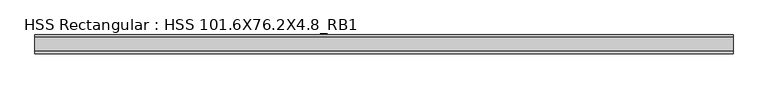
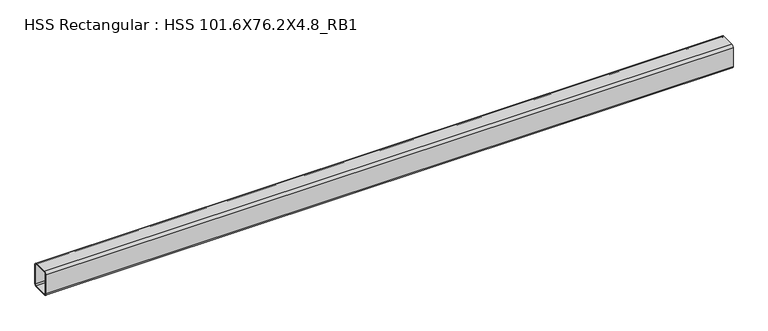
"""IFC4 building model written with IfcOpenShell, lengths in millimetres: beam geometry, HSS Rectangular : HSS 101.6X76.2X4.8_RB1."""

from ifc_helpers import new_model, si_unit, point, frame, frame_2d, origin, place, context, project, spatial, polyline, circle_curve, trimmed, segment, composite_curve, outline, extrude, source, transform, mapped, element, save


def hss_rectangular_hss_101_6x76_2x4_8_rb1_1d8725ce(model_context):
    return source(origin(), model_context, "Body", "SweptSolid", [
        extrude(outline(composite_curve([segment(trimmed(circle_curve(frame_2d((-28.575, 41.275)), 9.525), [point((-38.1, 41.275))], [point((-28.575, 50.8))], False, "CARTESIAN"), True, "CONTINUOUS"), segment(polyline([(-28.575, 50.8), (28.575, 50.8)]), True, "CONTINUOUS"), segment(trimmed(circle_curve(frame_2d((28.575, 41.275)), 9.525), [point((28.575, 50.8))], [point((38.1, 41.275))], False, "CARTESIAN"), True, "CONTINUOUS"), segment(polyline([(38.1, 41.275), (38.1, -41.275)]), True, "CONTINUOUS"), segment(trimmed(circle_curve(frame_2d((28.575, -41.275)), 9.525), [point((38.1, -41.275))], [point((28.575, -50.8))], False, "CARTESIAN"), True, "CONTINUOUS"), segment(polyline([(28.575, -50.8), (-28.575, -50.8)]), True, "CONTINUOUS"), segment(trimmed(circle_curve(frame_2d((-28.575, -41.275)), 9.525), [point((-28.575, -50.8))], [point((-38.1, -41.275))], False, "CARTESIAN"), True, "CONTINUOUS"), segment(polyline([(-38.1, -41.275), (-38.1, 41.275)]), True, "CONTINUOUS")], self_intersect=False), holes=[composite_curve([segment(polyline([(28.575, 46.0375), (-28.575, 46.0375)]), True, "CONTINUOUS"), segment(trimmed(circle_curve(frame_2d((-28.575, 41.275)), 4.7625), [point((-28.575, 46.0375))], [point((-33.3375, 41.275))], True, "CARTESIAN"), True, "CONTINUOUS"), segment(polyline([(-33.3375, 41.275), (-33.3375, -41.275)]), True, "CONTINUOUS"), segment(trimmed(circle_curve(frame_2d((-28.575, -41.275)), 4.7625), [point((-33.3375, -41.275))], [point((-28.575, -46.0375))], True, "CARTESIAN"), True, "CONTINUOUS"), segment(polyline([(-28.575, -46.0375), (28.575, -46.0375)]), True, "CONTINUOUS"), segment(trimmed(circle_curve(frame_2d((28.575, -41.275)), 4.7625), [point((28.575, -46.0375))], [point((33.3375, -41.275))], True, "CARTESIAN"), True, "CONTINUOUS"), segment(polyline([(33.3375, -41.275), (33.3375, 41.275)]), True, "CONTINUOUS"), segment(trimmed(circle_curve(frame_2d((28.575, 41.275)), 4.7625), [point((33.3375, 41.275))], [point((28.575, 46.0375))], True, "CARTESIAN"), True, "CONTINUOUS")], self_intersect=False)]), frame((-1442.3750006, 0.0, 0.0), z_axis=(1.0, 0.0, 0.0), x_axis=(0.0, 1.0, 0.0)), (0.0, 0.0, 1.0), 2827.6000006),
    ])


if __name__ == "__main__":
    model = new_model("IFC4")
    model_context = context("Model", 3, world=origin())
    ifc_project = project(units=[si_unit("LENGTHUNIT", "METRE", prefix="MILLI")], contexts=[model_context])
    site = spatial("IfcSite", under=ifc_project)
    building = spatial("IfcBuilding", under=site)
    placement = place(None, origin())
    hss_rectangular_hss_101_6x76_2x4_8_rb1_shape = hss_rectangular_hss_101_6x76_2x4_8_rb1_1d8725ce(model_context)
    element("IfcBeam", 1, ObjectType="HSS Rectangular : HSS 101.6X76.2X4.8_RB1", at=placement, inside=building, context=model_context, shape_type="MappedRepresentation", body=[
        mapped(hss_rectangular_hss_101_6x76_2x4_8_rb1_shape, transform((0.0, 0.0, 0.0), x_axis=(1.0, 0.0, 0.0), y_axis=(0.0, 1.0, 0.0), z_axis=(0.0, 0.0, 1.0))),
    ])
    save(model, "model.ifc")

# Revit data of these elements
# Type "HSS Rectangular : HSS 101.6X76.2X4.8_RB1"
#   Section Name Key = "HSS 4X3X3/16"
#   Assembly Code = "B10"
#   Width = 7.62 cm
#   Wall Nominal Thickness = 0.4763 cm
#   Wall Design Thickness = 0.442 cm
#   Torsional Moment of Inertia = 260.561 cm⁴
#   Torsional Modulus = 61.2876 cm³
#   Section Area = 14.4516 cm²
#   Plastic Modulus weak axis = 40.3122 cm³
#   Plastic Modulus strong axis = 49.1612 cm³
#   Perimeter = 0.881482 m²/m
#   Outer Fillet = 0.9525 cm
#   Nominal Weight = 12.1285 kgf/m
#   Moment of Inertia weak axis = 131.529 cm⁴
#   Moment of Inertia strong axis = 205.202 cm⁴
#   Inner Fillet = 0.4763 cm
#   Height = 10.16 cm
#   Elastic Modulus weak axis = 34.4128 cm³
#   Elastic Modulus strong axis = 40.476 cm³
#   Centroid Vertical = 5.08 cm
#   Centroid Horizontal = 3.81 cm
#   Length [instance default] = 1524 mm
#   Structural Material [instance default] = Steel ASTM A500, Grade B, Rectangular and Square
#   Principal Axes Angle = 0
# Element 1 (IfcBeam, "HSS Rectangular : HSS 101.6X76.2X4.8_RB1")
#   Structural Material = Steel ASTM A992
#   Materials on its faces: "Steel ASTM A992"
# Materials
#   "Steel ASTM A500, Grade B, Rectangular and Square": class "Metal", colour RGB 199 199 199, transparency 0, Description = "Carbon steel", Cost = 0
#   "Steel ASTM A992": class "Metal", colour RGB 199 199 199, transparency 0, Description = "Structural steel 50ksi", Cost = 0
